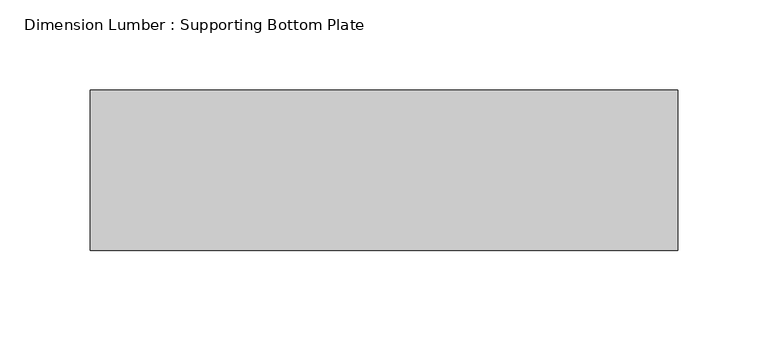
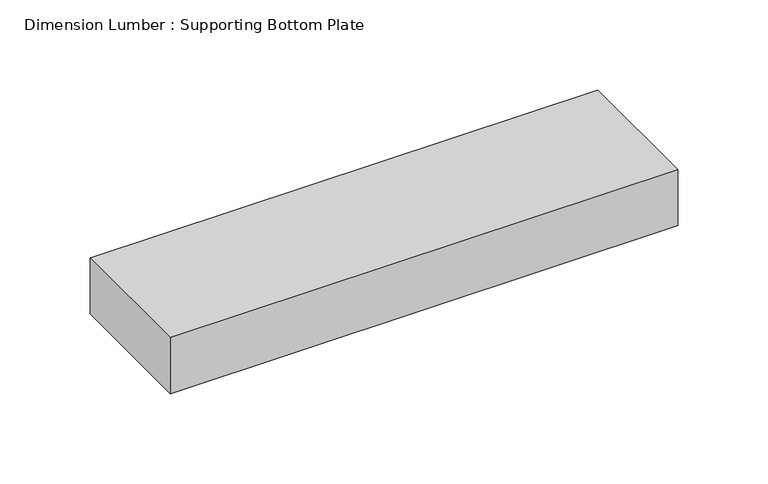
"""IFC4 building model written with IfcOpenShell, lengths in millimetres: beam geometry, Dimension Lumber : Supporting Bottom Plate."""

from ifc_helpers import new_model, si_unit, frame, origin, place, context, project, spatial, polyline, outline, extrude, source, transform, mapped, element, save


def dimension_lumber_supporting_bottom_plate_f7639587(model_context):
    return source(origin(), model_context, "Body", "SweptSolid", [
        extrude(outline(polyline([(184.9437503, 44.45), (184.9437503, -44.45), (-140.4937503, -44.45), (-140.4937503, 44.45), (184.9437503, 44.45)])), frame((0.0, 0.0, -19.05), z_axis=(0.0, 0.0, 1.0), x_axis=(1.0, 0.0, 0.0)), (0.0, 0.0, 1.0), 38.1),
    ])


if __name__ == "__main__":
    model = new_model("IFC4")
    model_context = context("Model", 3, world=origin())
    ifc_project = project(units=[si_unit("LENGTHUNIT", "METRE", prefix="MILLI")], contexts=[model_context])
    site = spatial("IfcSite", under=ifc_project)
    building = spatial("IfcBuilding", under=site)
    placement = place(None, origin())
    dimension_lumber_supporting_bottom_plate_shape = dimension_lumber_supporting_bottom_plate_f7639587(model_context)
    element("IfcBeam", 1, ObjectType="Dimension Lumber : Supporting Bottom Plate", at=placement, inside=building, context=model_context, shape_type="MappedRepresentation", body=[
        mapped(dimension_lumber_supporting_bottom_plate_shape, transform((0.0, 0.0, 0.0), x_axis=(1.0, 0.0, 0.0), y_axis=(0.0, 1.0, 0.0), z_axis=(0.0, 0.0, 1.0))),
    ])
    save(model, "model.ifc")

# Revit data of these elements
# Type "Dimension Lumber : Supporting Bottom Plate"
#   Assembly Code = "B10"
#   A = 0.0364583 SF
#   Length [instance default] = 5' - 0"
#   b = 0' - 3 1/2"
#   d = 0' - 1 1/2"
#   Structural Material [instance default] = Softwood, Lumber
# Element 1 (IfcBeam, "Dimension Lumber : Supporting Bottom Plate")
#   Structural Material = Douglas Fir #2
#   Materials on its faces: "Douglas Fir #2"
# Materials
#   "Softwood, Lumber": class "Wood", colour RGB 223 192 134, transparency 0, Description = "Pinus Echinata", Cost = 0
#   "Douglas Fir #2": class "Wood", colour RGB 223 192 134, transparency 0, Description = "Pinus Echinata", Cost = 0
